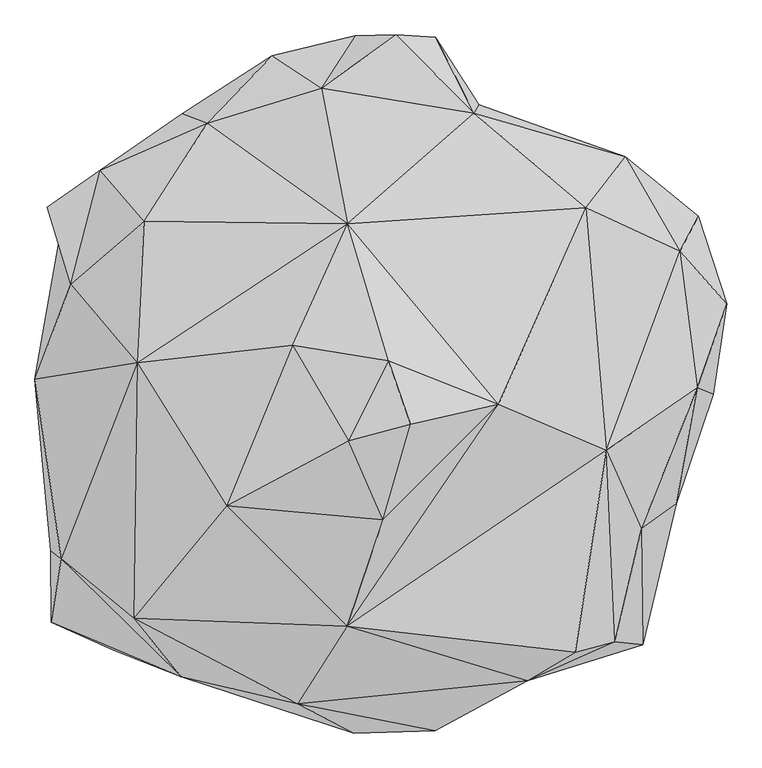
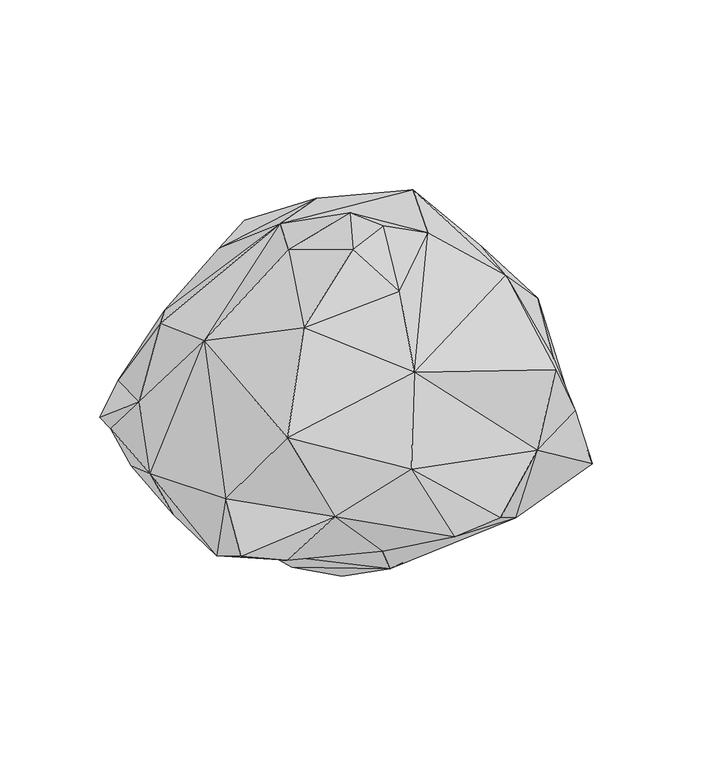
"""IFC4 building model written with IfcOpenShell, lengths in millimetres: geographic element geometry, Enscape AssetDefinition - Bush 061 Yeg : Enscape AssetDefinition - Bush 061 Yeg."""

import ifcopenshell
import ifcopenshell.guid

model = None  # the IFC model being written
_history = None  # IfcOwnerHistory: only IFC2X3 demands one
_inside = {}  # id of a spatial element -> (the spatial element, [elements in it])
_under = {}  # id of a project, library or spatial element -> (it, [spatial elements below it])
_declared = {}  # id of a project -> (the project, [libraries it declares])
_typed = {}  # id of a type object -> (the type object, [elements of that type])
_made_of = {}  # id of a material, layer set ... -> (it, [elements and type objects made of it])


def new_model(schema):
    """Start an empty IFC model of exactly this schema.

    Asked for "IFC4X3", IfcOpenShell would pick the latest addendum, in which some entities
    have other attributes; the version numbers below select the first issue.
    IFC2X3 requires an IfcOwnerHistory on every rooted entity: one is made here for all.
    """
    global model, _history
    if schema == "IFC4X3":
        model = ifcopenshell.file(schema_version=(4, 3, 0, 0))
    else:
        model = ifcopenshell.file(schema=schema)
    _inside.clear()
    _under.clear()
    _declared.clear()
    _typed.clear()
    _made_of.clear()
    _history = None
    if model.schema == "IFC2X3":
        org = make("IfcOrganization", Name="unknown")
        user = make(
            "IfcPersonAndOrganization",
            ThePerson=make("IfcPerson", FamilyName="unknown"),
            TheOrganization=org,
        )
        app = make(
            "IfcApplication",
            ApplicationDeveloper=org,
            Version="unknown",
            ApplicationFullName="unknown",
            ApplicationIdentifier="unknown",
        )
        _history = make(
            "IfcOwnerHistory",
            OwningUser=user,
            OwningApplication=app,
            ChangeAction="ADDED",
            CreationDate=0,
        )
    return model


def make(cls, **values):
    """One entity of the class cls with the attributes given. An attribute that is None is left unset."""
    return model.create_entity(
        cls, **{name: value for name, value in values.items() if value is not None}
    )


def rooted(cls, **values):
    """An entity with a GlobalId (a new one), such as an element, a storey or a relation."""
    return make(cls, GlobalId=ifcopenshell.guid.new(), OwnerHistory=_history, **values)


def si_unit(unit_type, name, prefix=None):
    """IfcSIUnit, for example si_unit("LENGTHUNIT", "METRE", prefix="MILLI")."""
    return make("IfcSIUnit", UnitType=unit_type, Prefix=prefix, Name=name)


def assignment(units):
    """IfcUnitAssignment: the units of a project."""
    return None if units is None else make("IfcUnitAssignment", Units=units)


def point(xyz):
    """IfcCartesianPoint."""
    return None if xyz is None else make("IfcCartesianPoint", Coordinates=xyz)


def direction(xyz):
    """IfcDirection."""
    return None if xyz is None else make("IfcDirection", DirectionRatios=xyz)


def frame(location, z_axis=None, x_axis=None):
    """IfcAxis2Placement3D, a coordinate frame: its origin and axes. An axis left out is left unset."""
    return make(
        "IfcAxis2Placement3D",
        Location=point(location),
        Axis=direction(z_axis),
        RefDirection=direction(x_axis),
    )


def origin():
    """The frame at (0, 0, 0) with its axes left unset."""
    return frame((0.0, 0.0, 0.0))


def place(relative_to, where):
    """IfcLocalPlacement: puts the frame where relative to a parent placement (None: the world)."""
    return make(
        "IfcLocalPlacement", PlacementRelTo=relative_to, RelativePlacement=where
    )


def context(
    kind, dimensions, precision=None, world=None, true_north=None, identifier=None
):
    """IfcGeometricRepresentationContext, for example the 3D "Model" context."""
    return make(
        "IfcGeometricRepresentationContext",
        ContextIdentifier=identifier,
        ContextType=kind,
        CoordinateSpaceDimension=dimensions,
        Precision=precision,
        WorldCoordinateSystem=world,
        TrueNorth=true_north,
    )


def project(units=None, contexts=None):
    """IfcProject with its units and contexts."""
    return rooted(
        "IfcProject",
        Name="project",
        RepresentationContexts=contexts,
        UnitsInContext=assignment(units),
    )


def spatial(cls, under=None, at=None, **own):
    """A site, building, storey or space (cls), placed at a placement, below another one or the project."""
    s = rooted(cls, ObjectPlacement=at, **own)
    if under is not None:
        _under.setdefault(under.id(), (under, []))[1].append(s)
    return s


def faces_of(points, faces, orient=None, outer=None):
    """IfcFace entities. A face is a list of loops; a loop is a list of indices into points, from 0.

    orient and outer hold one flag for each loop. By default every Orientation is true, the
    first loop of a face is its IfcFaceOuterBound and the others are IfcFaceBound.
    """
    made = []
    for i, loops in enumerate(faces):
        bounds = []
        for j, loop in enumerate(loops):
            is_outer = j == 0 if outer is None else outer[i][j]
            bounds.append(
                make(
                    "IfcFaceOuterBound" if is_outer else "IfcFaceBound",
                    Bound=make("IfcPolyLoop", Polygon=[points[k] for k in loop]),
                    Orientation=True if orient is None else orient[i][j],
                )
            )
        made.append(make("IfcFace", Bounds=bounds))
    return made


def faceted_brep(points, faces, orient=None, outer=None, voids=None):
    """IfcFacetedBrep: a solid bounded by flat faces; with voids (closed shells), ...WithVoids."""
    shared = [point(p) for p in points]
    hull = make("IfcClosedShell", CfsFaces=faces_of(shared, faces, orient, outer))
    if voids is None:
        return make("IfcFacetedBrep", Outer=hull)
    return make(
        "IfcFacetedBrepWithVoids",
        Outer=hull,
        Voids=[
            make(cls, CfsFaces=faces_of(shared, fs, o, b)) for cls, fs, o, b in voids
        ],
    )


def shape(context_of_items, identifier, shape_type, items):
    """IfcShapeRepresentation: the items that make up one representation, for example the "Body"."""
    return make(
        "IfcShapeRepresentation",
        ContextOfItems=context_of_items,
        RepresentationIdentifier=identifier,
        RepresentationType=shape_type,
        Items=items,
    )


def source(mapping_origin, context_of_items, identifier, shape_type, items):
    """IfcRepresentationMap: a shape defined once, which mapped items show again and again."""
    return make(
        "IfcRepresentationMap",
        MappingOrigin=mapping_origin,
        MappedRepresentation=shape(context_of_items, identifier, shape_type, items),
    )


def transform(
    local_origin,
    x_axis=None,
    y_axis=None,
    z_axis=None,
    scale=None,
    scale2=None,
    scale3=None,
    uniform=True,
):
    """IfcCartesianTransformationOperator3D, or its non-uniform kind. x_axis, y_axis, z_axis: its Axis1, 2, 3."""
    if uniform:
        return make(
            "IfcCartesianTransformationOperator3D",
            Axis1=direction(x_axis),
            Axis2=direction(y_axis),
            LocalOrigin=point(local_origin),
            Scale=scale,
            Axis3=direction(z_axis),
        )
    return make(
        "IfcCartesianTransformationOperator3DnonUniform",
        Axis1=direction(x_axis),
        Axis2=direction(y_axis),
        LocalOrigin=point(local_origin),
        Scale=scale,
        Axis3=direction(z_axis),
        Scale2=scale2,
        Scale3=scale3,
    )


def mapped(mapping_source, mapping_target):
    """IfcMappedItem: shows the shape of a source again, moved by a transform."""
    return make(
        "IfcMappedItem", MappingSource=mapping_source, MappingTarget=mapping_target
    )


def made_of(thing, what):
    """Note that an element or type object is made of a material, layer set ...; save() writes the relation."""
    if what is not None:
        _made_of.setdefault(what.id(), (what, []))[1].append(thing)
    return thing


def element(
    cls,
    number,
    at=None,
    inside=None,
    cuts=None,
    type_object=None,
    material=None,
    context=None,
    identifier="Body",
    shape_type=None,
    held_by="IfcProductDefinitionShape",
    body=None,
    shapes=None,
    **own,
):
    """One element of the class cls, such as IfcWall. Its Tag is "e" and its number.

    at: its placement. inside: the storey or other place that contains it. cuts: it is an
    opening in that element (IfcRelVoidsElement). A single representation is given by context,
    identifier, shape_type and body (its items); several are given by shapes. held_by: the class
    of the entity that holds the representations. save() writes the other relations.
    """
    e = rooted(cls, Tag="e%d" % number, ObjectPlacement=at, **own)
    if body is not None:
        shapes = [shape(context, identifier, shape_type, body)]
    if shapes is not None:
        e.Representation = make(held_by, Representations=shapes)
    if inside is not None:
        _inside.setdefault(inside.id(), (inside, []))[1].append(e)
    if cuts is not None:
        rooted(
            "IfcRelVoidsElement", RelatingBuildingElement=cuts, RelatedOpeningElement=e
        )
    if type_object is not None:
        _typed.setdefault(type_object.id(), (type_object, []))[1].append(e)
    return made_of(e, material)


def aggregate(whole, parts):
    """IfcRelAggregates: a whole, such as a stair, and the parts it consists of."""
    return rooted("IfcRelAggregates", RelatingObject=whole, RelatedObjects=parts)


def save(model, path):
    """Write the relations noted so far, then the file.

    IfcRelAggregates (storeys below a building ...), IfcRelContainedInSpatialStructure (elements
    in a storey), IfcRelDefinesByType, IfcRelAssociatesMaterial and IfcRelDeclares: one each for
    every whole, place, type object, material and project.
    """
    for whole, parts in _under.values():
        aggregate(whole, parts)
    for where, things in _inside.values():
        rooted(
            "IfcRelContainedInSpatialStructure",
            RelatedElements=things,
            RelatingStructure=where,
        )
    for kind, things in _typed.values():
        rooted("IfcRelDefinesByType", RelatedObjects=things, RelatingType=kind)
    for what, things in _made_of.values():
        rooted("IfcRelAssociatesMaterial", RelatedObjects=things, RelatingMaterial=what)
    for by, libraries in _declared.values():
        rooted("IfcRelDeclares", RelatingContext=by, RelatedDefinitions=libraries)
    model.write(path)


def geographic_element_7e854a61(model_context):
    return source(origin(), model_context, "Body", "Brep", [
        faceted_brep([(97.7892652, 98.1485918, 0.0), (160.0047797, -179.5626283, 37.216384), (-109.9038348, -103.1278893, 0.0), (-57.8008965, -356.4046323, 166.5240824), (350.6040275, -419.0308154, 283.9225233), (313.746959, -11.4472462, 92.0399651), (566.5103793, -201.2764812, 402.6556015), (-214.1610384, 178.9466441, 69.7101429), (-312.5149608, -93.0666253, 102.5632247), (-426.6794324, 474.8810828, 363.4885848), (26.8471297, 397.2656429, 172.8380173), (-531.193316, 151.2268633, 315.6976104), (-517.7954435, -281.9718719, 347.0107019), (-743.9683676, 315.4922724, 452.1919191), (-757.2122812, -9.7019263, 439.820677), (-240.1868552, -618.8186407, 467.4891531), (-639.5571828, -623.0279803, 569.2309737), (-792.1186686, -383.7651014, 498.5969067), (-829.7457099, 29.0031135, 620.3073263), (-757.6228976, 439.8719966, 543.5131788), (-766.1955357, -403.5795927, 750.1796484), (-583.6555362, 68.7348172, 1092.8783417), (-743.2497144, 258.5127056, 766.4521337), (-790.9380198, -556.7570925, 600.8008122), (-476.5750468, -687.4508262, 741.812408), (-592.0741558, -547.157824, 1045.2927351), (-60.3675433, -823.1237531, 592.1768546), (-196.3485032, -752.3869872, 891.1912441), (-77.6667446, -565.3297305, 1162.6911163), (-367.6465452, -275.0932574, 1283.0156088), (357.3286235, -696.7420578, 748.1776476), (134.4409883, -817.6311255, 603.0080914), (294.5484519, -649.721086, 445.3133047), (636.1178756, -610.6053591, 538.739264), (472.879082, -628.4692287, 1017.9835558), (568.8202977, -602.5974154, 790.0140285), (717.0186043, -270.2166438, 651.1070728), (632.2165728, -330.840826, 842.4249291), (547.9278564, -141.2682682, 1112.3849154), (767.1709061, 8.5212691, 843.1949615), (498.6995459, 442.5926507, 1149.7552395), (287.3618305, -31.2617645, 1323.3119249), (724.7185111, 337.5654221, 884.9286437), (805.9785962, -6.5706167, 655.9323668), (838.8829827, 211.5430534, 728.8764715), (769.3268657, 422.3674536, 650.2857208), (593.7681794, 565.8430457, 786.8313789), (229.098931, 670.0489521, 1068.1359768), (-75.8700892, 403.9902687, 1224.5987654), (240.9055084, 691.0440922, 677.1329045), (607.6280475, 489.7162914, 523.4933496), (747.2023368, 248.6567795, 554.0878177), (425.652802, 244.0368235, 281.4585567), (291.1604643, 494.5415854, 385.0997388), (-125.9197146, 718.7638879, 457.2225213), (-56.9795705, 823.9964247, 560.6584549), (-257.9993904, 808.3398938, 657.1130157), (-57.4415661, 856.9008708, 700.4893422), (-474.6757448, 668.7655449, 557.5784445), (-672.7696061, 533.297956, 669.4329381), (-414.8728549, 646.384418, 816.5531158), (-139.0096098, 730.9811711, 941.3436055), (-566.2024021, 409.7909033, 957.9241276), (-799.6646166, 443.4653223, 607.0120931), (23.3564898, 73.2007772, 1439.1191006), (-208.1037611, 111.6491556, 1333.5784674), (-73.5601112, -118.9384311, 1429.9818277), (76.2294233, -79.2580694, 1456.8289518), (9.8045925, -309.1783226, 1330.7038546), (41.3230211, 858.8514924, 924.3522882), (136.0836327, 853.7695408, 876.8180609)], [[[0, 1, 2]], [[2, 1, 3]], [[1, 4, 3]], [[5, 6, 1]], [[1, 0, 5]], [[1, 6, 4]], [[7, 0, 2]], [[2, 3, 8]], [[2, 8, 7]], [[7, 9, 10]], [[7, 11, 9]], [[7, 8, 11]], [[10, 0, 7]], [[3, 12, 8]], [[12, 11, 8]], [[9, 11, 13]], [[11, 12, 14]], [[11, 14, 13]], [[12, 15, 16]], [[12, 16, 17]], [[3, 15, 12]], [[14, 12, 17]], [[14, 18, 13]], [[14, 17, 18]], [[13, 18, 19]], [[9, 13, 19]], [[17, 20, 18]], [[20, 21, 18]], [[18, 21, 22]], [[18, 22, 19]], [[17, 23, 20]], [[17, 16, 23]], [[23, 24, 20]], [[20, 25, 21]], [[24, 25, 20]], [[16, 24, 23]], [[15, 24, 16]], [[15, 26, 24]], [[26, 27, 24]], [[24, 27, 25]], [[25, 27, 28]], [[25, 29, 21]], [[25, 28, 29]], [[30, 28, 27]], [[26, 31, 27]], [[31, 30, 27]], [[32, 31, 26]], [[32, 26, 15]], [[3, 32, 15]], [[4, 33, 32]], [[4, 32, 3]], [[32, 33, 30]], [[32, 30, 31]], [[34, 28, 30]], [[30, 33, 35]], [[35, 34, 30]], [[4, 6, 33]], [[6, 36, 33]], [[33, 37, 35]], [[36, 37, 33]], [[37, 38, 35]], [[38, 34, 35]], [[34, 38, 28]], [[38, 37, 39]], [[40, 41, 38]], [[38, 41, 28]], [[39, 42, 38]], [[42, 40, 38]], [[36, 39, 37]], [[43, 39, 36]], [[6, 43, 36]], [[43, 44, 39]], [[44, 42, 39]], [[45, 42, 44]], [[46, 40, 42]], [[46, 42, 45]], [[46, 47, 40]], [[47, 48, 40]], [[40, 48, 41]], [[46, 49, 47]], [[50, 49, 46]], [[50, 46, 45]], [[51, 45, 44]], [[45, 51, 50]], [[51, 44, 43]], [[51, 43, 6]], [[52, 50, 51]], [[52, 51, 6]], [[53, 49, 50]], [[50, 52, 53]], [[5, 52, 6]], [[0, 52, 5]], [[0, 10, 52]], [[10, 53, 52]], [[54, 49, 53]], [[10, 54, 53]], [[10, 9, 54]], [[54, 55, 49]], [[54, 56, 57]], [[58, 56, 54]], [[54, 9, 58]], [[54, 57, 55]], [[9, 19, 58]], [[58, 59, 60]], [[19, 59, 58]], [[58, 60, 56]], [[56, 61, 57]], [[56, 60, 61]], [[60, 62, 48]], [[60, 48, 61]], [[59, 62, 60]], [[19, 63, 59]], [[22, 62, 59]], [[63, 22, 59]], [[19, 22, 63]], [[22, 21, 62]], [[62, 21, 48]], [[48, 64, 41]], [[48, 65, 64]], [[61, 48, 47]], [[48, 21, 65]], [[21, 29, 65]], [[65, 29, 66]], [[65, 66, 64]], [[66, 67, 64]], [[41, 64, 67]], [[68, 28, 41]], [[41, 67, 68]], [[66, 68, 67]], [[66, 29, 68]], [[28, 68, 29]], [[69, 61, 47]], [[57, 61, 69]], [[57, 69, 70]], [[69, 47, 70]], [[49, 70, 47]], [[57, 70, 49]], [[55, 57, 49]]]),
    ])


if __name__ == "__main__":
    model = new_model("IFC4")
    model_context = context("Model", 3, world=origin())
    ifc_project = project(units=[si_unit("LENGTHUNIT", "METRE", prefix="MILLI")], contexts=[model_context])
    site = spatial("IfcSite", under=ifc_project)
    building = spatial("IfcBuilding", under=site)
    placement = place(None, origin())
    geographic_element_shape = geographic_element_7e854a61(model_context)
    element("IfcGeographicElement", 1, ObjectType="Enscape AssetDefinition - Bush 061 Yeg : Enscape AssetDefinition - Bush 061 Yeg", at=placement, inside=building, context=model_context, shape_type="MappedRepresentation", body=[
        mapped(geographic_element_shape, transform((0.0, 0.0, 0.0), x_axis=(1.0, 0.0, 0.0), y_axis=(0.0, 1.0, 0.0), z_axis=(0.0, 0.0, 1.0))),
    ])
    save(model, "model.ifc")

# Revit data of these elements
# Type "Enscape AssetDefinition - Bush 061 Yeg : Enscape AssetDefinition - Bush 061 Yeg"
#   EnscapeAssetSource = "REMOTE"
#   EnscapeAssetId = "c6641aa6-f25d-4e4a-b8f4-059183b6f3ff"
#   Height = 1456.829 mm
#   EnscapeNativeAssetHeight = 1456.829 mm
#   Default Elevation = 0
